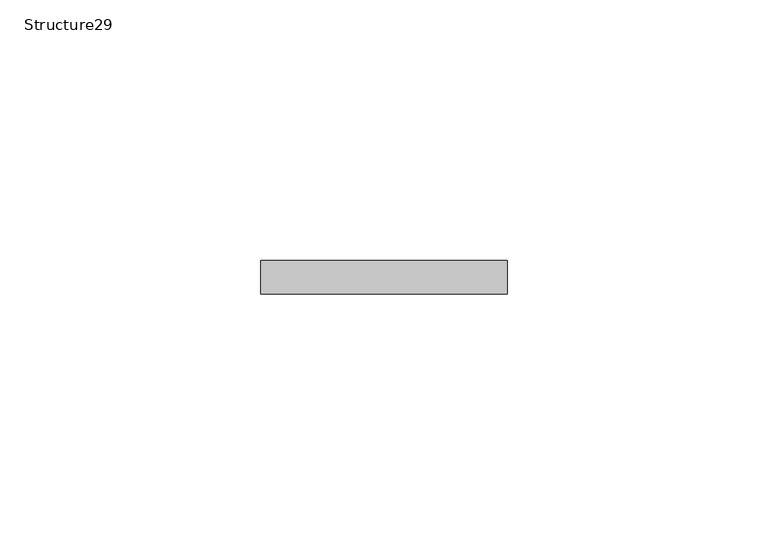
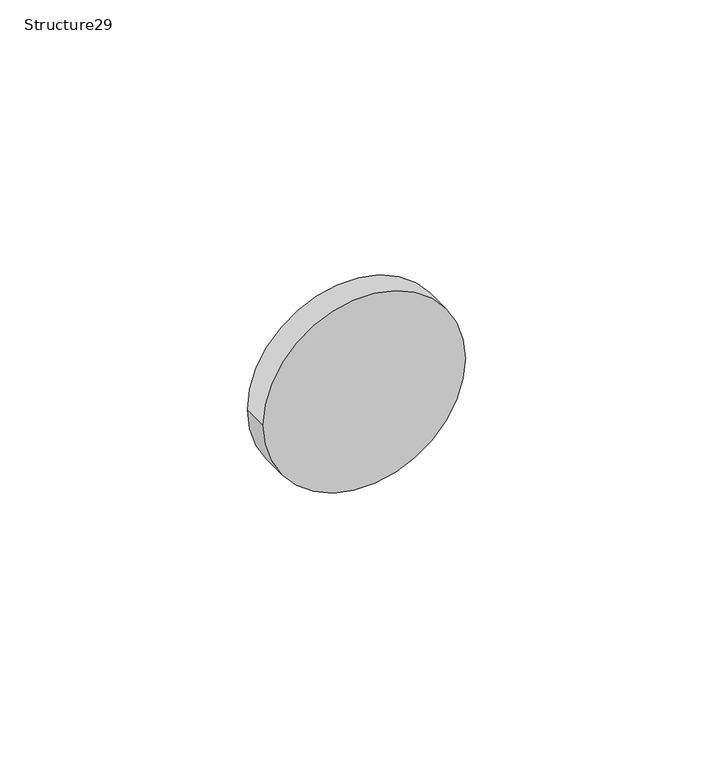
"""IFC4 building model written with IfcOpenShell, lengths in millimetres: proxy geometry, Structure29 : Structure668217127."""

from ifc_helpers import new_model, si_unit, point, frame, frame_2d, origin, place, context, project, spatial, circle_curve, trimmed, segment, composite_curve, outline, extrude, source, transform, mapped, element, save


def structure29_ad517188(model_context):
    return source(origin(), model_context, "Body", "SweptSolid", [
        extrude(outline(composite_curve([segment(trimmed(circle_curve(frame_2d((38047.8454063, 5185.7383658)), 23.5716554), [point((38047.8454063, 5162.1667104))], [point((38047.8454063, 5209.3100213))], False, "CARTESIAN"), True, "CONTINUOUS"), segment(trimmed(circle_curve(frame_2d((38047.8454063, 5185.7383658)), 23.5716554), [point((38047.8454063, 5209.3100213))], [point((38047.8454063, 5162.1667104))], False, "CARTESIAN"), True, "CONTINUOUS")], self_intersect=False)), frame((0.0, 916.5010696, 0.0), z_axis=(0.0, 1.0, 0.0), x_axis=(0.0, 0.0, 1.0)), (0.0, 0.0, 1.0), 6.35),
    ])


if __name__ == "__main__":
    model = new_model("IFC4")
    model_context = context("Model", 3, world=origin())
    ifc_project = project(units=[si_unit("LENGTHUNIT", "METRE", prefix="MILLI")], contexts=[model_context])
    site = spatial("IfcSite", under=ifc_project)
    building = spatial("IfcBuilding", under=site)
    placement = place(None, origin())
    structure29_shape = structure29_ad517188(model_context)
    element("IfcBuildingElementProxy", 1, Name="Structure29 : Structure668217127", ObjectType="Structure29 : Structure668217127", at=placement, inside=building, context=model_context, shape_type="MappedRepresentation", body=[
        mapped(structure29_shape, transform((0.0, 0.0, 0.0), x_axis=(1.0, 0.0, 0.0), y_axis=(0.0, 1.0, 0.0), z_axis=(0.0, 0.0, 1.0))),
    ])
    save(model, "model.ifc")

# Revit data of these elements
# Type "Structure29 : Structure668217127"
#   NameOverride = "Structure668217127"
# Element 1 (IfcBuildingElementProxy, "Structure29 : Structure668217127")
#   Materials on its faces: "RUBBER GASKET"
# Materials
#   "RUBBER GASKET": class "Unassigned", colour RGB 70 70 70, transparency 0
